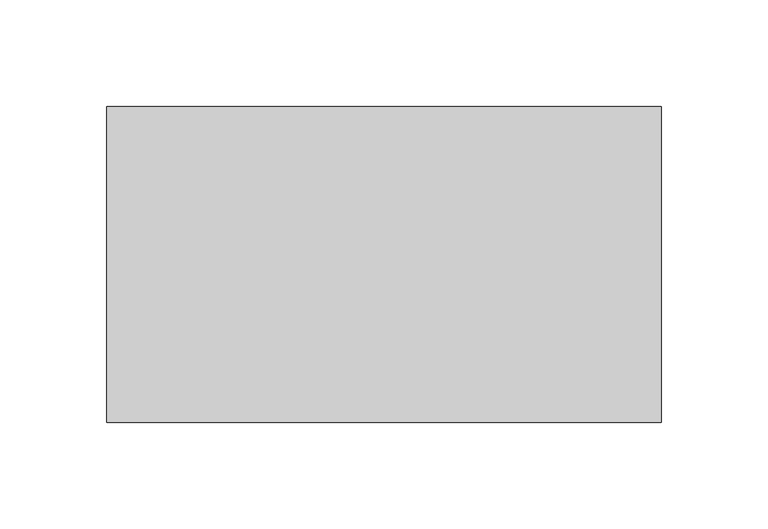
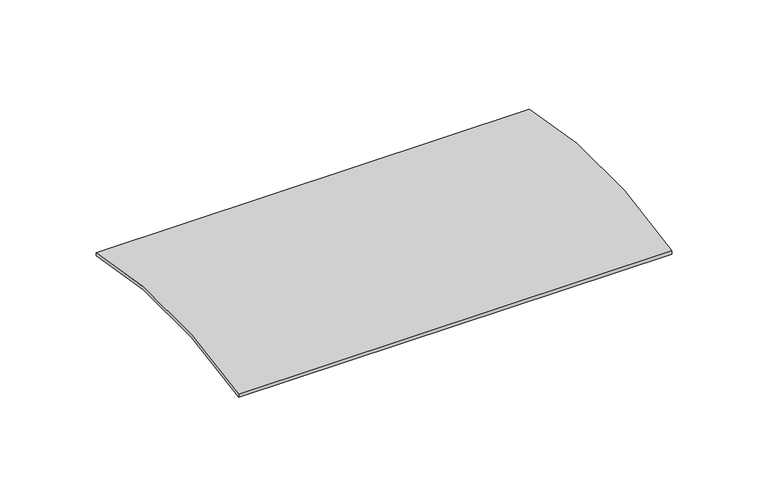
"""IFC4 building model written with IfcOpenShell, lengths in millimetres: proxy geometry, TN_ПВС 125-82_Защитная решетка : TN_ПВС 125-82_Защитная решетка."""

from ifc_helpers import new_model, si_unit, point, frame, frame_2d, origin, place, context, project, spatial, polyline, circle_curve, trimmed, segment, composite_curve, outline, extrude, source, transform, mapped, element, save


def generic_models_7c4a537d(model_context):
    return source(origin(), model_context, "Body", "SweptSolid", [
        extrude(outline(composite_curve([segment(trimmed(circle_curve(frame_2d((0.0, -288.7046439)), 298.0), [point((74.1, -0.0644007))], [point((-74.1, -0.0644007))], True, "CARTESIAN"), True, "CONTINUOUS"), segment(polyline([(-74.1, -0.0644007), (-74.1, 2.0)]), True, "CONTINUOUS"), segment(trimmed(circle_curve(frame_2d((0.0, -288.7046439)), 300.0), [point((-74.1, 2.0))], [point((74.1, 2.0))], False, "CARTESIAN"), True, "CONTINUOUS"), segment(polyline([(74.1, 2.0), (74.1, -0.0644007)]), True, "CONTINUOUS")], self_intersect=False)), frame((0.0, 0.0, 0.0), z_axis=(1.0, 0.0, 0.0), x_axis=(0.0, 1.0, 0.0)), (0.0, 0.0, 1.0), 260.0),
    ])


if __name__ == "__main__":
    model = new_model("IFC4")
    model_context = context("Model", 3, world=origin())
    ifc_project = project(units=[si_unit("LENGTHUNIT", "METRE", prefix="MILLI")], contexts=[model_context])
    site = spatial("IfcSite", under=ifc_project)
    building = spatial("IfcBuilding", under=site)
    placement = place(None, origin())
    generic_models_shape = generic_models_7c4a537d(model_context)
    element("IfcBuildingElementProxy", 1, Name="TN_ПВС 125-82_Защитная решетка : TN_ПВС 125-82_Защитная решетка", ObjectType="TN_ПВС 125-82_Защитная решетка : TN_ПВС 125-82_Защитная решетка", at=placement, inside=building, context=model_context, shape_type="MappedRepresentation", body=[
        mapped(generic_models_shape, transform((0.0, 0.0, 0.0), x_axis=(1.0, 0.0, 0.0), y_axis=(0.0, 1.0, 0.0), z_axis=(0.0, 0.0, 1.0))),
    ])
    save(model, "model.ifc")

# Revit data of these elements
# Type "TN_ПВС 125-82_Защитная решетка : TN_ПВС 125-82_Защитная решетка"
#   Description = "Служит для предотвращения засора водосточной системы. Не пропускает в желоб листья и прочий крупный\r\nмусор"
#   Manufacturer = "ТехноНИКОЛЬ"
#   Model = "Комплектующие к водосточным системам"
#   URL = "https://tn-vodostok.ru/catalog/pvh/"
#   ADSK_Обозначение = "ТехноНИКОЛЬ"
#   ADSK_Наименование краткое = "Решетка"
#   ADSK_Наименование = "Защитная решетка"
#   ADSK_Масса_Текст = ""
#   ADSK_Марка = ""
#   ADSK_Код изделия = ""
#   ADSK_Завод-изготовитель = "ТехноНИКОЛЬ"
#   ADSK_Единица измерения = "п.м."
#   ADSK_Группирование = "Комплектующие к водосточным системам"
#   ADSK_URL страницы изделия = "https://tn-vodostok.ru/catalog/pvh/"
#   ADSK_URL документации изделия = "https://tn-vodostok.ru/upload/iblock/c42/c427963cb77eb5c3c51f0cfb870e9e52.pdf"
#   ADSK_Размер_Длина [instance default] = 500 mm
#   ADSK_Количество [instance default] = 0.5
#   ADSK_Материал [instance default] = TN_Пластик_Решетка_Коричневый_RAL8019
#   Default Elevation = 0
# Element 1 (IfcBuildingElementProxy, "TN_ПВС 125-82_Защитная решетка : TN_ПВС 125-82_Защитная решетка")
#   ADSK_Размер_Длина = 260 mm
#   ADSK_Количество = 0.26
#   Materials on its faces: "TN_Пластик_Решетка_Коричневый_RAL8019"
# Materials
#   "TN_Пластик_Решетка_Коричневый_RAL8019": class "Типовые", colour RGB 61 54 53, transparency 0.25, Cost = 0
